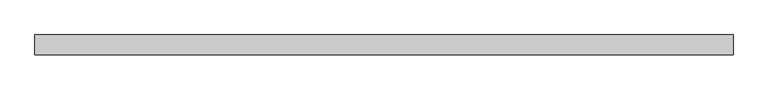
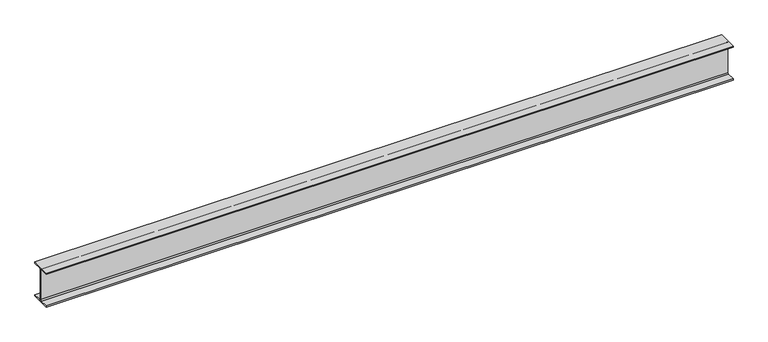
"""IFC4 building model written with IfcOpenShell, lengths in millimetres: beam geometry, Old_Steel Beam_H-KSD3502 : H_SB_ASB_H-400×200x8x13."""

from ifc_helpers import new_model, si_unit, point, frame, frame_2d, origin, place, context, project, spatial, polyline, circle_curve, trimmed, segment, composite_curve, outline, extrude, source, transform, mapped, element, save


def beam_3cb43d04(model_context):
    return source(origin(), model_context, "Body", "SweptSolid", [
        extrude(outline(composite_curve([segment(polyline([(82.5, -141.5), (82.5, -151.7), (-82.5, -151.7), (-82.5, -141.5), (-11.9, -141.5)]), True, "CONTINUOUS"), segment(trimmed(circle_curve(frame_2d((-11.9, -132.6)), 8.9), [point((-11.9, -141.5))], [point((-3.0, -132.6))], True, "CARTESIAN"), True, "CONTINUOUS"), segment(polyline([(-3.0, -132.6), (-3.0, 132.6)]), True, "CONTINUOUS"), segment(trimmed(circle_curve(frame_2d((-11.9, 132.6)), 8.9), [point((-3.0, 132.6))], [point((-11.9, 141.5))], True, "CARTESIAN"), True, "CONTINUOUS"), segment(polyline([(-11.9, 141.5), (-82.5, 141.5), (-82.5, 151.7), (82.5, 151.7), (82.5, 141.5), (11.9, 141.5)]), True, "CONTINUOUS"), segment(trimmed(circle_curve(frame_2d((11.9, 132.6)), 8.9), [point((11.9, 141.5))], [point((3.0, 132.6))], True, "CARTESIAN"), True, "CONTINUOUS"), segment(polyline([(3.0, 132.6), (3.0, -132.6)]), True, "CONTINUOUS"), segment(trimmed(circle_curve(frame_2d((11.9, -132.6)), 8.9), [point((3.0, -132.6))], [point((11.9, -141.5))], True, "CARTESIAN"), True, "CONTINUOUS"), segment(polyline([(11.9, -141.5), (82.5, -141.5)]), True, "CONTINUOUS")], self_intersect=False)), frame((-2904.8, 0.0, 0.0), z_axis=(1.0, 0.0, 0.0), x_axis=(0.0, 1.0, 0.0)), (0.0, 0.0, 1.0), 5809.6),
    ])


if __name__ == "__main__":
    model = new_model("IFC4")
    model_context = context("Model", 3, world=origin())
    ifc_project = project(units=[si_unit("LENGTHUNIT", "METRE", prefix="MILLI")], contexts=[model_context])
    site = spatial("IfcSite", under=ifc_project)
    building = spatial("IfcBuilding", under=site)
    placement = place(None, origin())
    beam_shape = beam_3cb43d04(model_context)
    element("IfcBeam", 1, ObjectType="Old_Steel Beam_H-KSD3502 : H_SB_ASB_H-400×200x8x13", at=placement, inside=building, context=model_context, shape_type="MappedRepresentation", body=[
        mapped(beam_shape, transform((0.0, 0.0, 0.0), x_axis=(1.0, 0.0, 0.0), y_axis=(0.0, 1.0, 0.0), z_axis=(0.0, 0.0, 1.0))),
    ])
    save(model, "model.ifc")

# Revit data of these elements
# Type "Old_Steel Beam_H-KSD3502 : H_SB_ASB_H-400×200x8x13"
#   Width = 20.0 cm
#   Web Thickness = 0.8 cm
#   Web Fillet = 1.6 cm
#   Warping Constant = 648999.0 cm⁶
#   Torsional Moment of Inertia = 35.8981 cm⁴
#   Torsional Modulus = 1.0 cm³
#   Section Area = 84.12 cm²
#   Plastic Modulus weak axis = 268.0 cm³
#   Plastic Modulus strong axis = 1330.0 cm³
#   Perimeter = 1.56 m²/m
#   Nominal Weight = 66.00 kgf/m
#   Moment of Inertia weak axis = 1740.00 cm⁴
#   Moment of Inertia strong axis = 23700.00 cm⁴
#   Height = 40.0 cm
#   Flange Thickness = 1.3 cm
#   Elastic Modulus weak axis = 174.0 cm³
#   Elastic Modulus strong axis = 1190.0 cm³
#   Centroid Vertical = 20.0 cm
#   Centroid Horizontal = 10.0 cm
#   Length [instance default] = 1.5240 m
#   Structural Material [instance default] = Steel, 45-345
#   Assembly Code = ""
# Element 1 (IfcBeam, "Old_Steel Beam_H-KSD3502 : H_SB_ASB_H-400×200x8x13")
#   Structural Material = none
# Materials
#   "Steel, 45-345": class "Metal", colour RGB 189 187 185, transparency 0, Description = "Steel 345 MPa", Cost = 0
